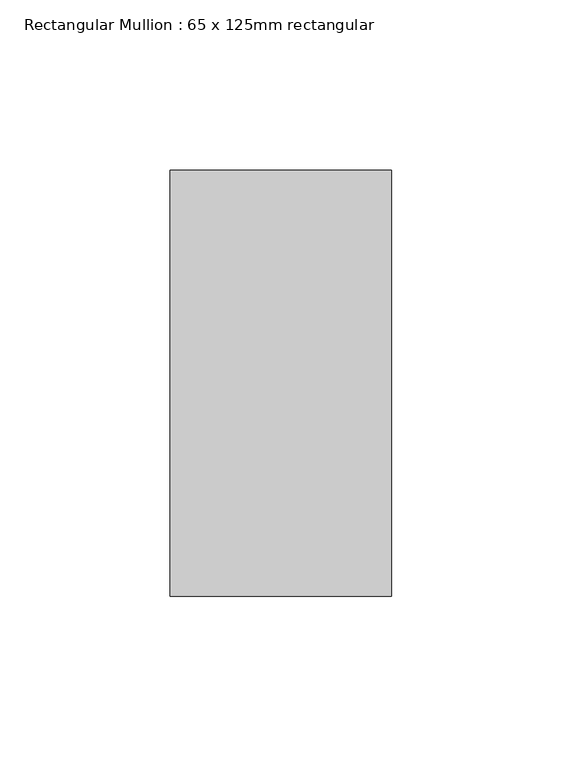
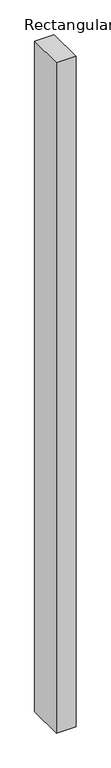
"""IFC4 building model written with IfcOpenShell, lengths in millimetres: member geometry, Rectangular Mullion : 65 x 125mm rectangular."""

from ifc_helpers import new_model, si_unit, frame, origin, place, context, project, spatial, polyline, outline, extrude, source, transform, mapped, element, save


def rectangular_mullion_65_x_125mm_rectangular_617b4e42(model_context):
    return source(origin(), model_context, "Body", "SweptSolid", [
        extrude(outline(polyline([(0.0, 62.5), (0.0, -62.5), (-65.0, -62.5), (-65.0, 62.5), (0.0, 62.5)])), frame((0.0, 0.0, -2355.6422537), z_axis=(0.0, 0.0, 1.0), x_axis=(1.0, 0.0, 0.0)), (0.0, 0.0, 1.0), 2355.6422537),
    ])


if __name__ == "__main__":
    model = new_model("IFC4")
    model_context = context("Model", 3, world=origin())
    ifc_project = project(units=[si_unit("LENGTHUNIT", "METRE", prefix="MILLI")], contexts=[model_context])
    site = spatial("IfcSite", under=ifc_project)
    building = spatial("IfcBuilding", under=site)
    placement = place(None, origin())
    rectangular_mullion_65_x_125mm_rectangular_shape = rectangular_mullion_65_x_125mm_rectangular_617b4e42(model_context)
    element("IfcMember", 1, ObjectType="Rectangular Mullion : 65 x 125mm rectangular", at=placement, inside=building, context=model_context, shape_type="MappedRepresentation", body=[
        mapped(rectangular_mullion_65_x_125mm_rectangular_shape, transform((0.0, 0.0, 0.0), x_axis=(1.0, 0.0, 0.0), y_axis=(0.0, 1.0, 0.0), z_axis=(0.0, 0.0, 1.0))),
    ])
    save(model, "model.ifc")

# Revit data of these elements
# Type "Rectangular Mullion : 65 x 125mm rectangular"
#   built-in parameter 1007304 = 0.410105 (stored number, unit not read)
#   built-in parameter 1007301 = 0.106627 (stored number, unit not read)
#   built-in parameter 1007300 = 0.106627 (stored number, unit not read)
# Element 1 (IfcMember, "Rectangular Mullion : 65 x 125mm rectangular")
#   Materials on its faces: "Aluminum"
# Materials
#   "Aluminum": class "Metal", colour RGB 244 245 246, transparency 0, Description = "Aluminum 6061", Cost = 0
